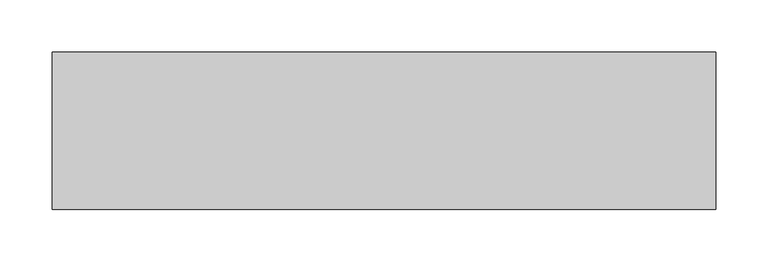
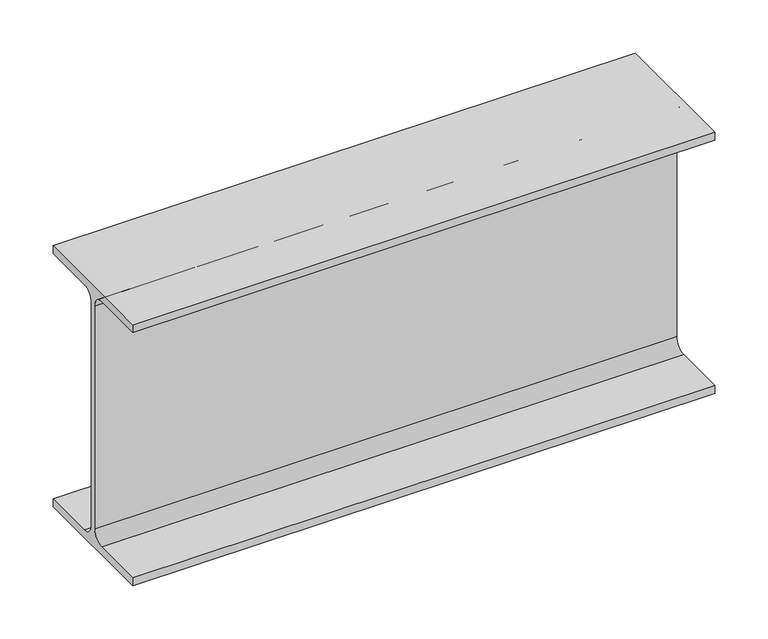
"""IFC4 building model written with IfcOpenShell, lengths in millimetres: beam geometry, 0912_Steel Framing_H-KSD3502 : H_SB_ASB_H-300x150x6.5x9."""

from ifc_helpers import new_model, si_unit, point, frame, frame_2d, origin, place, context, project, spatial, polyline, circle_curve, trimmed, segment, composite_curve, outline, extrude, source, transform, mapped, element, save


def beam_d6a3fa63(model_context):
    return source(origin(), model_context, "Body", "SweptSolid", [
        extrude(outline(composite_curve([segment(polyline([(75.0, -141.0), (75.0, -150.0), (-75.0, -150.0), (-75.0, -141.0), (-16.25, -141.0)]), True, "CONTINUOUS"), segment(trimmed(circle_curve(frame_2d((-16.25, -128.0)), 13.0), [point((-16.25, -141.0))], [point((-3.25, -128.0))], True, "CARTESIAN"), True, "CONTINUOUS"), segment(polyline([(-3.25, -128.0), (-3.25, 128.0)]), True, "CONTINUOUS"), segment(trimmed(circle_curve(frame_2d((-16.25, 128.0)), 13.0), [point((-3.25, 128.0))], [point((-16.25, 141.0))], True, "CARTESIAN"), True, "CONTINUOUS"), segment(polyline([(-16.25, 141.0), (-75.0, 141.0), (-75.0, 150.0), (75.0, 150.0), (75.0, 141.0), (16.25, 141.0)]), True, "CONTINUOUS"), segment(trimmed(circle_curve(frame_2d((16.25, 128.0)), 13.0), [point((16.25, 141.0))], [point((3.25, 128.0))], True, "CARTESIAN"), True, "CONTINUOUS"), segment(polyline([(3.25, 128.0), (3.25, -128.0)]), True, "CONTINUOUS"), segment(trimmed(circle_curve(frame_2d((16.25, -128.0)), 13.0), [point((3.25, -128.0))], [point((16.25, -141.0))], True, "CARTESIAN"), True, "CONTINUOUS"), segment(polyline([(16.25, -141.0), (75.0, -141.0)]), True, "CONTINUOUS")], self_intersect=False)), frame((-238.55, 0.0, 0.0), z_axis=(1.0, 0.0, 0.0), x_axis=(0.0, 1.0, 0.0)), (0.0, 0.0, 1.0), 632.1),
    ])


if __name__ == "__main__":
    model = new_model("IFC4")
    model_context = context("Model", 3, world=origin())
    ifc_project = project(units=[si_unit("LENGTHUNIT", "METRE", prefix="MILLI")], contexts=[model_context])
    site = spatial("IfcSite", under=ifc_project)
    building = spatial("IfcBuilding", under=site)
    placement = place(None, origin())
    beam_shape = beam_d6a3fa63(model_context)
    element("IfcBeam", 1, ObjectType="0912_Steel Framing_H-KSD3502 : H_SB_ASB_H-300x150x6.5x9", at=placement, inside=building, context=model_context, shape_type="MappedRepresentation", body=[
        mapped(beam_shape, transform((0.0, 0.0, 0.0), x_axis=(1.0, 0.0, 0.0), y_axis=(0.0, 1.0, 0.0), z_axis=(0.0, 0.0, 1.0))),
    ])
    save(model, "model.ifc")

# Revit data of these elements
# Type "0912_Steel Framing_H-KSD3502 : H_SB_ASB_H-300x150x6.5x9"
#   H_WM Code_1 = "S01AA002-00001 | Main Steel Structure Fabrication Work | Shelter/Building | Medium Steel - Standard (90KG/M>Weight≥30KG/M) | Material: (   )"
#   H_WM Code_2 = "S03AA028-00001 | Main Steel Structure Erection Work | Shelter/Building | Medium Steel (90KG/M>Weight≥30KG/M) | Material: (   )"
#   H_WM Code_3 = "S01AA010-00001 | Main Steel Structure Fabrication Work | Shelter/Building | Steel Painting/Coating | for Non-Fireproofed Steel Surface, Surface Preparation, Primer, Second & Final Coat | Material: (   )"
#   H_Q'ty Cal Type Tag = "SB-Q2"
#   Width = 15.0 cm
#   Web Thickness = 0.65 cm
#   Web Fillet = 1.3 cm
#   Warping Constant = 107000.0 cm⁶
#   W = 0
#   Torsional Moment of Inertia = 9.9539 cm⁴
#   Section Area = 46.78 cm²
#   Plastic Modulus weak axis = 105.0 cm³
#   Plastic Modulus strong axis = 542.0 cm³
#   Perimeter = 1.17 m²/m
#   Nominal Weight = 36.70 kgf/m
#   Moment of Inertia weak axis = 508.00 cm⁴
#   Moment of Inertia strong axis = 7210.00 cm⁴
#   Height = 30.0 cm
#   Flange Thickness = 0.9 cm
#   Elastic Modulus weak axis = 67.7 cm³
#   Elastic Modulus strong axis = 481.0 cm³
#   Centroid Vertical = 15.0 cm
#   Centroid Horizontal = 7.5 cm
#   Ix = 72100000
#   Length [instance default] = 1.5240 m
#   Zx = 542000
#   b = 0.1500 m
#   h = 0.3000 m
#   r = 0.0130 m
#   s = 0.0065 m
#   t = 0.0090 m
#   A = 0.004678 m²
#   Structural Material [instance default] = Steel, 45-345
#   Assembly Code = ""
# Element 1 (IfcBeam, "0912_Steel Framing_H-KSD3502 : H_SB_ASB_H-300x150x6.5x9")
#   Structural Material = none
# Materials
#   "Steel, 45-345": class "Metal", colour RGB 189 187 185, transparency 0, Description = "Steel 345 MPa", Cost = 0
